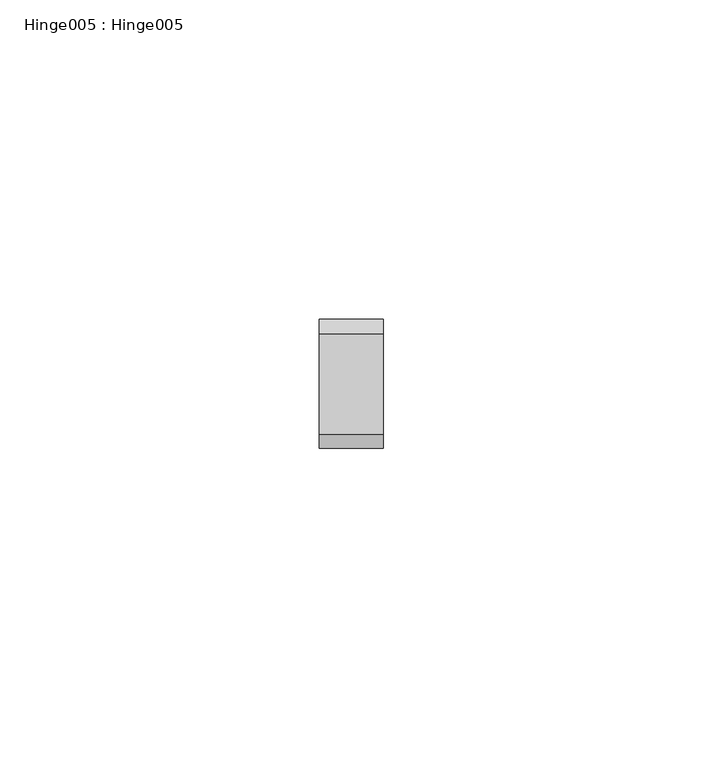
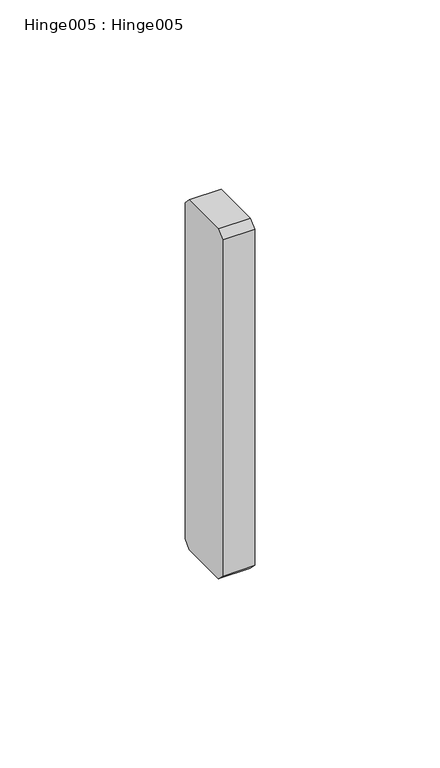
"""IFC4 building model written with IfcOpenShell, lengths in millimetres: proxy geometry, Hinge005 : Hinge005."""

from ifc_helpers import new_model, si_unit, frame, origin, place, context, project, spatial, polyline, outline, extrude, source, transform, mapped, element, save


def hinge005_hinge005_3f589e26(model_context):
    return source(origin(), model_context, "Body", "SweptSolid", [
        extrude(outline(polyline([(9646.679882, 39394.6012561), (9630.9579547, 39394.6012561), (9628.7124545, 39396.8467563), (9628.7124545, 39507.7452438), (9630.9579547, 39509.9907439), (9646.679882, 39509.9907439), (9648.924946, 39507.7456799), (9648.924946, 39396.8463201), (9646.679882, 39394.6012561)])), frame((-7242.2219278, 0.0, 0.0), z_axis=(1.0, 0.0, 0.0), x_axis=(0.0, 1.0, 0.0)), (0.0, 0.0, 1.0), 10.0),
    ])


if __name__ == "__main__":
    model = new_model("IFC4")
    model_context = context("Model", 3, world=origin())
    ifc_project = project(units=[si_unit("LENGTHUNIT", "METRE", prefix="MILLI")], contexts=[model_context])
    site = spatial("IfcSite", under=ifc_project)
    building = spatial("IfcBuilding", under=site)
    placement = place(None, origin())
    hinge005_hinge005_shape = hinge005_hinge005_3f589e26(model_context)
    element("IfcBuildingElementProxy", 1, Name="Hinge005 : Hinge005", ObjectType="Hinge005 : Hinge005", at=placement, inside=building, context=model_context, shape_type="MappedRepresentation", body=[
        mapped(hinge005_hinge005_shape, transform((0.0, 0.0, 0.0), x_axis=(1.0, 0.0, 0.0), y_axis=(0.0, 1.0, 0.0), z_axis=(0.0, 0.0, 1.0))),
    ])
    save(model, "model.ifc")

# Revit data of these elements
# Type "Hinge005 : Hinge005"
#   NameOverride = "Hinge005"
# Element 1 (IfcBuildingElementProxy, "Hinge005 : Hinge005")
#   Materials on its faces: "HEAVY DUTY STAINLESS STEEL HINGE (90 DEGREE ROTATION)"
# Materials
#   "HEAVY DUTY STAINLESS STEEL HINGE (90 DEGREE ROTATION)": class "Unassigned", colour RGB 128 128 128, transparency 0
